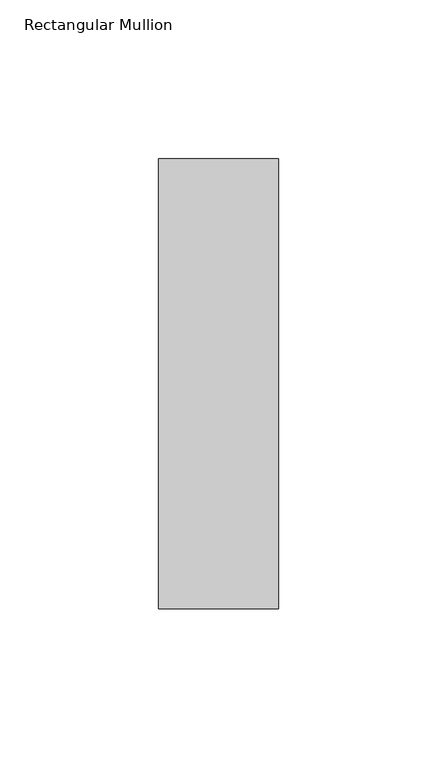
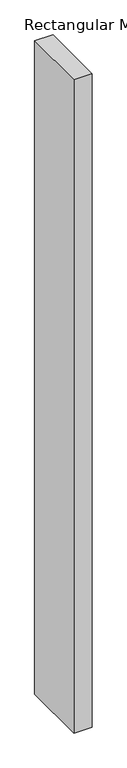
"""IFC4 building model written with IfcOpenShell, lengths in millimetres: member geometry, Rectangular Mullion : NLRS_21_CWM_hsb-regel 38x142_gen_rsf."""

from ifc_helpers import new_model, si_unit, frame, origin, place, context, project, spatial, polyline, outline, extrude, source, transform, mapped, element, save


def rectangular_mullion_878a7b4c(model_context):
    return source(origin(), model_context, "Body", "SweptSolid", [
        extrude(outline(polyline([(19.0, -71.0), (-19.0, -71.0), (-19.0, 71.0), (19.0, 71.0), (19.0, -71.0)])), frame((0.0, 0.0, -1440.0), z_axis=(0.0, 0.0, 1.0), x_axis=(1.0, 0.0, 0.0)), (0.0, 0.0, 1.0), 1440.0),
    ])


if __name__ == "__main__":
    model = new_model("IFC4")
    model_context = context("Model", 3, world=origin())
    ifc_project = project(units=[si_unit("LENGTHUNIT", "METRE", prefix="MILLI")], contexts=[model_context])
    site = spatial("IfcSite", under=ifc_project)
    building = spatial("IfcBuilding", under=site)
    placement = place(None, origin())
    rectangular_mullion_shape = rectangular_mullion_878a7b4c(model_context)
    element("IfcMember", 1, ObjectType="Rectangular Mullion : NLRS_21_CWM_hsb-regel 38x142_gen_rsf", at=placement, inside=building, context=model_context, shape_type="MappedRepresentation", body=[
        mapped(rectangular_mullion_shape, transform((0.0, 0.0, 0.0), x_axis=(1.0, 0.0, 0.0), y_axis=(0.0, 1.0, 0.0), z_axis=(0.0, 0.0, 1.0))),
    ])
    save(model, "model.ifc")

# Revit data of these elements
# Type "Rectangular Mullion : NLRS_21_CWM_hsb-regel 38x142_gen_rsf"
#   Export Type to IFC As = "IfcWall"
#   Type IfcGUID = "07M7mRoiH1CR8m_RSKIwpF"
#   Assembly Code = "21.10"
#   built-in parameter 1007322 = 0.465879 (stored number, unit not read)
#   built-in parameter 1007321 = 0.062336 (stored number, unit not read)
#   built-in parameter 1007320 = 0.062336 (stored number, unit not read)
# Element 1 (IfcMember, "Rectangular Mullion : NLRS_21_CWM_hsb-regel 38x142_gen_rsf")
#   Materials on its faces: "NLRS_i2_hout naaldhout vuren_gen_rsf"
# Materials
#   "NLRS_i2_hout naaldhout vuren_gen_rsf": class "I - Hout", colour RGB 234 199 147, transparency 0, Keynote = "i2", Manufacturer = "Revit Standards Foundation", URL = "www.revitstandards.org", Description = "hout vuren", Cost = 0
